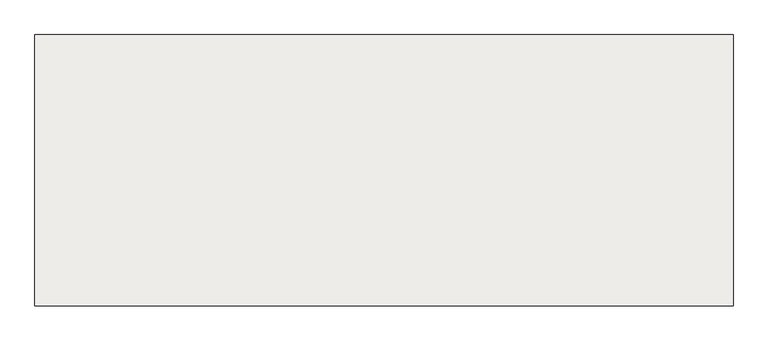
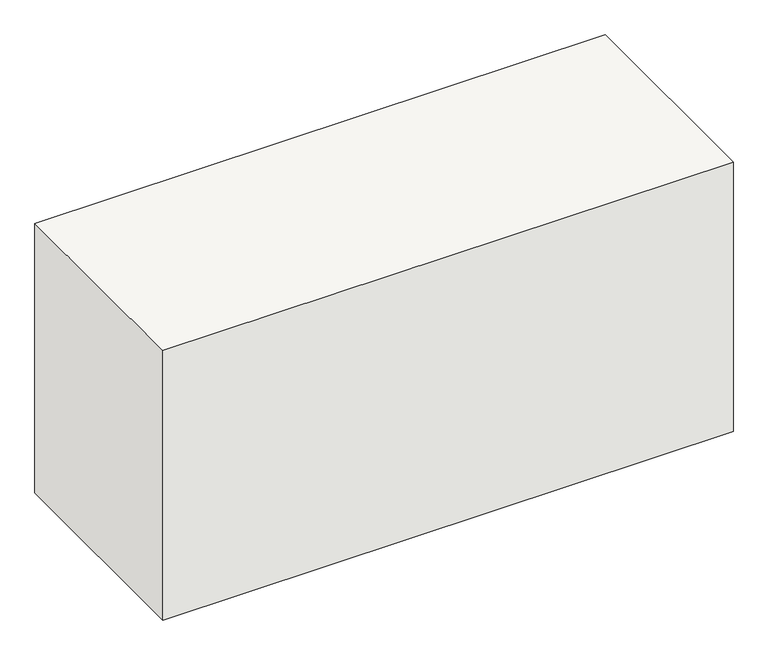
"""IFC4 building model written with IfcOpenShell, lengths in millimetres: slab geometry, NLRS_16_SFO_LB_funderingspoer meerpaals beton ihwg-MMBC-SH_gen_rsf : funderingspoer beton ihwg_gen__2-paals bxlxh 700x1800x1200."""

from ifc_helpers import new_model, si_unit, frame, origin, place, context, project, spatial, polyline, outline, extrude, source, transform, mapped, element, save


def slab_ec8fc613(model_context):
    return source(origin(), model_context, "Body", "SweptSolid", [
        extrude(outline(polyline([(900.0, 350.0), (900.0, -350.0), (-900.0, -350.0), (-900.0, 350.0), (900.0, 350.0)])), frame((0.0, 0.0, -1200.0), z_axis=(0.0, 0.0, 1.0), x_axis=(1.0, 0.0, 0.0)), (0.0, 0.0, 1.0), 900.0),
    ])


if __name__ == "__main__":
    model = new_model("IFC4")
    model_context = context("Model", 3, world=origin())
    ifc_project = project(units=[si_unit("LENGTHUNIT", "METRE", prefix="MILLI")], contexts=[model_context])
    site = spatial("IfcSite", under=ifc_project)
    building = spatial("IfcBuilding", under=site)
    placement = place(None, origin())
    slab_shape = slab_ec8fc613(model_context)
    element("IfcSlab", 1, ObjectType="NLRS_16_SFO_LB_funderingspoer meerpaals beton ihwg-MMBC-SH_gen_rsf : funderingspoer beton ihwg_gen__2-paals bxlxh 700x1800x1200", at=placement, inside=building, context=model_context, shape_type="MappedRepresentation", body=[
        mapped(slab_shape, transform((0.0, 0.0, 0.0), x_axis=(1.0, 0.0, 0.0), y_axis=(0.0, 1.0, 0.0), z_axis=(0.0, 0.0, 1.0))),
    ])
    save(model, "model.ifc")

# Revit data of these elements
# Type "NLRS_16_SFO_LB_funderingspoer meerpaals beton ihwg-MMBC-SH_gen_rsf : funderingspoer beton ihwg_gen__2-paals bxlxh 700x1800x1200"
#   Export Type to IFC As = "IfcFootingType"
#   Type IfcGUID = "1GXoSzV6T12eGHLrhjoRVK"
#   Type Comments = "2-paals poer 700x1800x1200"
#   Model = " "
#   Manufacturer = " "
#   Description = "2-paals poer 700x1800x1200"
#   Assembly Code = "16.13"
#   Width = 700 mm
#   Rough Height = 1200 mm
#   NLRS_C_lengte = 1800 mm
#   NLRS_C_hoogte = 1200 mm
#   NLRS_C_breedte = 700 mm
#   Length = 1800 mm
#   Height [instance default] = 1050 mm
#   Foundation Thickness = 1200 mm
#   Depth [instance default] = 150 mm
#   Structural Material = NLRS_f2_beton ihwg_gen_rsf
#   Keynote = ""
# Element 1 (IfcSlab, "NLRS_16_SFO_LB_funderingspoer meerpaals beton ihwg-MMBC-SH_gen_rsf : funderingspoer beton ihwg_gen__2-paals bxlxh 700x1800x1200")
#   Height = 900 mm
#   Depth = 300 mm
#   Materials on its faces: "NLRS_f2_beton ihwg_gen_rsf"
# Materials
#   "NLRS_f2_beton ihwg_gen_rsf": class "F - Niet gebakken kunststeen", colour RGB 129 133 118, transparency 0, Keynote = "f2", Manufacturer = "Revit Standards Foundation", URL = "www.revitstandards.org", Description = "beton ihwg", Cost = 0
